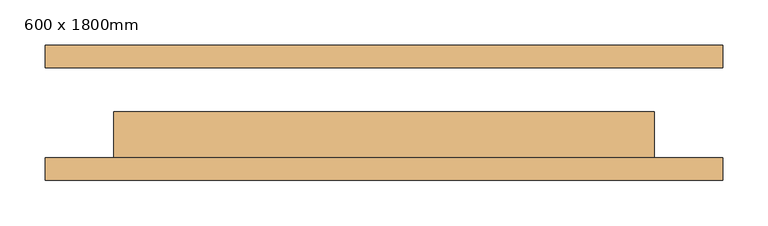
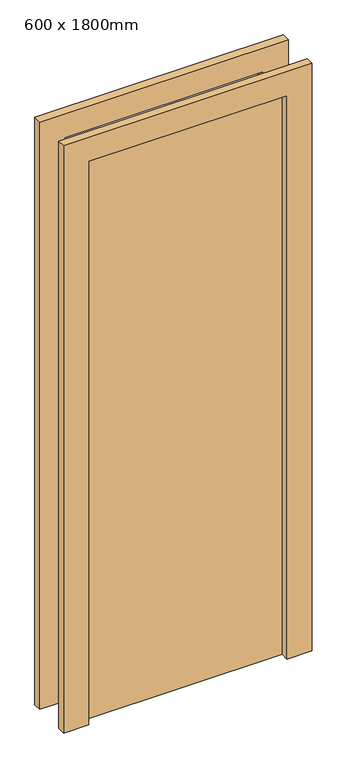
"""IFC4 building model written with IfcOpenShell, lengths in millimetres: door geometry, 单扇 - 与墙齐 : 600 x 1800mm."""

import ifcopenshell
import ifcopenshell.guid

model = None  # the IFC model being written
_history = None  # IfcOwnerHistory: only IFC2X3 demands one
_inside = {}  # id of a spatial element -> (the spatial element, [elements in it])
_under = {}  # id of a project, library or spatial element -> (it, [spatial elements below it])
_declared = {}  # id of a project -> (the project, [libraries it declares])
_typed = {}  # id of a type object -> (the type object, [elements of that type])
_made_of = {}  # id of a material, layer set ... -> (it, [elements and type objects made of it])


def new_model(schema):
    """Start an empty IFC model of exactly this schema.

    Asked for "IFC4X3", IfcOpenShell would pick the latest addendum, in which some entities
    have other attributes; the version numbers below select the first issue.
    IFC2X3 requires an IfcOwnerHistory on every rooted entity: one is made here for all.
    """
    global model, _history
    if schema == "IFC4X3":
        model = ifcopenshell.file(schema_version=(4, 3, 0, 0))
    else:
        model = ifcopenshell.file(schema=schema)
    _inside.clear()
    _under.clear()
    _declared.clear()
    _typed.clear()
    _made_of.clear()
    _history = None
    if model.schema == "IFC2X3":
        org = make("IfcOrganization", Name="unknown")
        user = make(
            "IfcPersonAndOrganization",
            ThePerson=make("IfcPerson", FamilyName="unknown"),
            TheOrganization=org,
        )
        app = make(
            "IfcApplication",
            ApplicationDeveloper=org,
            Version="unknown",
            ApplicationFullName="unknown",
            ApplicationIdentifier="unknown",
        )
        _history = make(
            "IfcOwnerHistory",
            OwningUser=user,
            OwningApplication=app,
            ChangeAction="ADDED",
            CreationDate=0,
        )
    return model


def make(cls, **values):
    """One entity of the class cls with the attributes given. An attribute that is None is left unset."""
    return model.create_entity(
        cls, **{name: value for name, value in values.items() if value is not None}
    )


def rooted(cls, **values):
    """An entity with a GlobalId (a new one), such as an element, a storey or a relation."""
    return make(cls, GlobalId=ifcopenshell.guid.new(), OwnerHistory=_history, **values)


def si_unit(unit_type, name, prefix=None):
    """IfcSIUnit, for example si_unit("LENGTHUNIT", "METRE", prefix="MILLI")."""
    return make("IfcSIUnit", UnitType=unit_type, Prefix=prefix, Name=name)


def assignment(units):
    """IfcUnitAssignment: the units of a project."""
    return None if units is None else make("IfcUnitAssignment", Units=units)


def point(xyz):
    """IfcCartesianPoint."""
    return None if xyz is None else make("IfcCartesianPoint", Coordinates=xyz)


def direction(xyz):
    """IfcDirection."""
    return None if xyz is None else make("IfcDirection", DirectionRatios=xyz)


def frame(location, z_axis=None, x_axis=None):
    """IfcAxis2Placement3D, a coordinate frame: its origin and axes. An axis left out is left unset."""
    return make(
        "IfcAxis2Placement3D",
        Location=point(location),
        Axis=direction(z_axis),
        RefDirection=direction(x_axis),
    )


def origin():
    """The frame at (0, 0, 0) with its axes left unset."""
    return frame((0.0, 0.0, 0.0))


def origin_with_axes():
    """The frame at (0, 0, 0) with the z axis (0, 0, 1) and the x axis (1, 0, 0) written out."""
    return frame((0.0, 0.0, 0.0), z_axis=(0.0, 0.0, 1.0), x_axis=(1.0, 0.0, 0.0))


def place(relative_to, where):
    """IfcLocalPlacement: puts the frame where relative to a parent placement (None: the world)."""
    return make(
        "IfcLocalPlacement", PlacementRelTo=relative_to, RelativePlacement=where
    )


def context(
    kind, dimensions, precision=None, world=None, true_north=None, identifier=None
):
    """IfcGeometricRepresentationContext, for example the 3D "Model" context."""
    return make(
        "IfcGeometricRepresentationContext",
        ContextIdentifier=identifier,
        ContextType=kind,
        CoordinateSpaceDimension=dimensions,
        Precision=precision,
        WorldCoordinateSystem=world,
        TrueNorth=true_north,
    )


def project(units=None, contexts=None):
    """IfcProject with its units and contexts."""
    return rooted(
        "IfcProject",
        Name="project",
        RepresentationContexts=contexts,
        UnitsInContext=assignment(units),
    )


def spatial(cls, under=None, at=None, **own):
    """A site, building, storey or space (cls), placed at a placement, below another one or the project."""
    s = rooted(cls, ObjectPlacement=at, **own)
    if under is not None:
        _under.setdefault(under.id(), (under, []))[1].append(s)
    return s


def polyline(points):
    """IfcPolyline through the points."""
    return make("IfcPolyline", Points=[point(p) for p in points])


def outline(outer, holes=None, kind="AREA"):
    """IfcArbitraryClosedProfileDef: a profile drawn as a closed curve; with holes, ...WithVoids."""
    if holes is None:
        return make("IfcArbitraryClosedProfileDef", ProfileType=kind, OuterCurve=outer)
    return make(
        "IfcArbitraryProfileDefWithVoids",
        ProfileType=kind,
        OuterCurve=outer,
        InnerCurves=holes,
    )


def extrude(swept, where, along, depth):
    """IfcExtrudedAreaSolid: the profile swept, set in the frame where, extruded along a direction by depth."""
    return make(
        "IfcExtrudedAreaSolid",
        SweptArea=swept,
        Position=where,
        ExtrudedDirection=direction(along),
        Depth=depth,
    )


def shape(context_of_items, identifier, shape_type, items):
    """IfcShapeRepresentation: the items that make up one representation, for example the "Body"."""
    return make(
        "IfcShapeRepresentation",
        ContextOfItems=context_of_items,
        RepresentationIdentifier=identifier,
        RepresentationType=shape_type,
        Items=items,
    )


def source(mapping_origin, context_of_items, identifier, shape_type, items):
    """IfcRepresentationMap: a shape defined once, which mapped items show again and again."""
    return make(
        "IfcRepresentationMap",
        MappingOrigin=mapping_origin,
        MappedRepresentation=shape(context_of_items, identifier, shape_type, items),
    )


def transform(
    local_origin,
    x_axis=None,
    y_axis=None,
    z_axis=None,
    scale=None,
    scale2=None,
    scale3=None,
    uniform=True,
):
    """IfcCartesianTransformationOperator3D, or its non-uniform kind. x_axis, y_axis, z_axis: its Axis1, 2, 3."""
    if uniform:
        return make(
            "IfcCartesianTransformationOperator3D",
            Axis1=direction(x_axis),
            Axis2=direction(y_axis),
            LocalOrigin=point(local_origin),
            Scale=scale,
            Axis3=direction(z_axis),
        )
    return make(
        "IfcCartesianTransformationOperator3DnonUniform",
        Axis1=direction(x_axis),
        Axis2=direction(y_axis),
        LocalOrigin=point(local_origin),
        Scale=scale,
        Axis3=direction(z_axis),
        Scale2=scale2,
        Scale3=scale3,
    )


def mapped(mapping_source, mapping_target):
    """IfcMappedItem: shows the shape of a source again, moved by a transform."""
    return make(
        "IfcMappedItem", MappingSource=mapping_source, MappingTarget=mapping_target
    )


def made_of(thing, what):
    """Note that an element or type object is made of a material, layer set ...; save() writes the relation."""
    if what is not None:
        _made_of.setdefault(what.id(), (what, []))[1].append(thing)
    return thing


def element(
    cls,
    number,
    at=None,
    inside=None,
    cuts=None,
    type_object=None,
    material=None,
    context=None,
    identifier="Body",
    shape_type=None,
    held_by="IfcProductDefinitionShape",
    body=None,
    shapes=None,
    **own,
):
    """One element of the class cls, such as IfcWall. Its Tag is "e" and its number.

    at: its placement. inside: the storey or other place that contains it. cuts: it is an
    opening in that element (IfcRelVoidsElement). A single representation is given by context,
    identifier, shape_type and body (its items); several are given by shapes. held_by: the class
    of the entity that holds the representations. save() writes the other relations.
    """
    e = rooted(cls, Tag="e%d" % number, ObjectPlacement=at, **own)
    if body is not None:
        shapes = [shape(context, identifier, shape_type, body)]
    if shapes is not None:
        e.Representation = make(held_by, Representations=shapes)
    if inside is not None:
        _inside.setdefault(inside.id(), (inside, []))[1].append(e)
    if cuts is not None:
        rooted(
            "IfcRelVoidsElement", RelatingBuildingElement=cuts, RelatedOpeningElement=e
        )
    if type_object is not None:
        _typed.setdefault(type_object.id(), (type_object, []))[1].append(e)
    return made_of(e, material)


def aggregate(whole, parts):
    """IfcRelAggregates: a whole, such as a stair, and the parts it consists of."""
    return rooted("IfcRelAggregates", RelatingObject=whole, RelatedObjects=parts)


def save(model, path):
    """Write the relations noted so far, then the file.

    IfcRelAggregates (storeys below a building ...), IfcRelContainedInSpatialStructure (elements
    in a storey), IfcRelDefinesByType, IfcRelAssociatesMaterial and IfcRelDeclares: one each for
    every whole, place, type object, material and project.
    """
    for whole, parts in _under.values():
        aggregate(whole, parts)
    for where, things in _inside.values():
        rooted(
            "IfcRelContainedInSpatialStructure",
            RelatedElements=things,
            RelatingStructure=where,
        )
    for kind, things in _typed.values():
        rooted("IfcRelDefinesByType", RelatedObjects=things, RelatingType=kind)
    for what, things in _made_of.values():
        rooted("IfcRelAssociatesMaterial", RelatedObjects=things, RelatingMaterial=what)
    for by, libraries in _declared.values():
        rooted("IfcRelDeclares", RelatingContext=by, RelatedDefinitions=libraries)
    model.write(path)


def door_600_x_1800mm_26a27b96(model_context):
    return source(origin(), model_context, "Body", "SweptSolid", [
        extrude(outline(polyline([(1876.0, -376.0), (0.0, -376.0), (0.0, -300.0), (1800.0, -300.0), (1800.0, 300.0), (0.0, 300.0), (0.0, 376.0), (1876.0, 376.0), (1876.0, -376.0)])), frame((0.0, -75.0, 0.0), z_axis=(0.0, 1.0, 0.0), x_axis=(0.0, 0.0, 1.0)), (0.0, 0.0, 1.0), 25.0),
        extrude(outline(polyline([(1876.0, 376.0), (1876.0, -376.0), (0.0, -376.0), (0.0, -300.0), (1800.0, -300.0), (1800.0, 300.0), (0.0, 300.0), (0.0, 376.0), (1876.0, 376.0)])), frame((0.0, 50.0, 0.0), z_axis=(0.0, 1.0, 0.0), x_axis=(0.0, 0.0, 1.0)), (0.0, 0.0, 1.0), 25.0),
        extrude(outline(polyline([(300.0, 1.0), (300.0, -50.0), (-300.0, -50.0), (-300.0, 1.0), (300.0, 1.0)])), origin_with_axes(), (0.0, 0.0, 1.0), 1800.0),
    ])


if __name__ == "__main__":
    model = new_model("IFC4")
    model_context = context("Model", 3, world=origin())
    ifc_project = project(units=[si_unit("LENGTHUNIT", "METRE", prefix="MILLI")], contexts=[model_context])
    site = spatial("IfcSite", under=ifc_project)
    building = spatial("IfcBuilding", under=site)
    placement = place(None, origin())
    door_600_x_1800mm_shape = door_600_x_1800mm_26a27b96(model_context)
    element("IfcDoor", 1, ObjectType="单扇 - 与墙齐 : 600 x 1800mm", at=placement, inside=building, context=model_context, shape_type="MappedRepresentation", body=[
        mapped(door_600_x_1800mm_shape, transform((0.0, 0.0, 0.0), x_axis=(1.0, 0.0, 0.0), y_axis=(0.0, 1.0, 0.0), z_axis=(0.0, 0.0, 1.0))),
    ])
    save(model, "model.ifc")

# Revit data of these elements
# Project information
#   项目发布日期 = "出图日期"
#   项目状态 = "项目状态"
#   客户姓名 = "所有者"
#   项目地址 = "请在此处输入地址"
#   项目名称 = "项目名称"
#   项目编号 = "项目编号"
# Type "单扇 - 与墙齐 : 600 x 1800mm"
#   Type Mark = "M0618"
#   Construction Type Id = "MDOOR"
#   Analytic Construction = "金属"
#   贴面宽度 = 76 mm
#   贴面投影内部 = 25 mm
#   贴面投影外部 = 25 mm
#   Thickness = 51 mm
#   Height = 1800 mm
#   Width = 600 mm
#   Heat Transfer Coefficient (U) = 3.7021 W/(m²·K)
#   框架材质 = 门 - 框架
#   门材质 = 门 - 嵌板
#   Visual Light Transmittance = 0
#   Solar Heat Gain Coefficient = 0
#   Wall Closure = (empty or 0)
#   Function = (empty or 0)
# Element 1 (IfcDoor, "单扇 - 与墙齐 : 600 x 1800mm")
#   Materials on its faces: "门 - 框架", "门 - 嵌板"
# Materials
#   "门 - 框架": class "其他", colour RGB 118 70 51, transparency 0, Cost = 0
#   "门 - 嵌板": class "木质", colour RGB 210 159 95, transparency 0, Cost = 0
